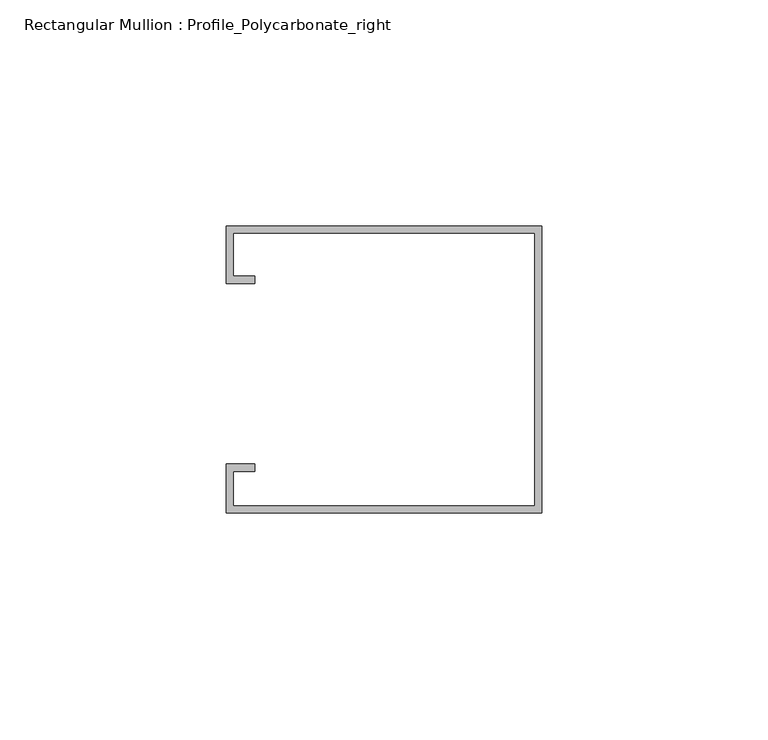
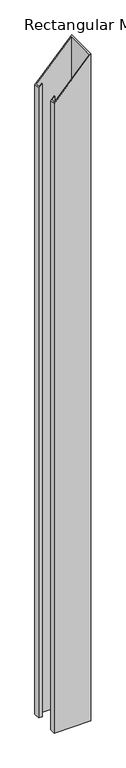
"""IFC4 building model written with IfcOpenShell, lengths in millimetres: member geometry, Rectangular Mullion : Profile_Polycarbonate_right."""

from ifc_helpers import new_model, si_unit, origin, place, context, project, spatial, faceted_brep, source, transform, mapped, element, save


def rectangular_mullion_profile_polycarbonate_right_a4e2f6aa(model_context):
    return source(origin(), model_context, "Body", "Brep", [
        faceted_brep([(0.0, 32.7, -1345.3170334), (0.0, -30.8, -1345.3170334), (-69.85, -30.8, -1345.3170334), (-69.85, -20.0, -1345.3170334), (-63.5, -20.0, -1345.3170334), (-63.5, -21.5875, -1345.3170334), (-68.2625, -21.5875, -1345.3170334), (-68.2625, -29.2125, -1345.3170334), (-1.5875, -29.2125, -1345.3170334), (-1.5875, 31.1125, -1345.3170334), (-68.2625, 31.1125, -1345.3170334), (-68.2625, 21.5875, -1345.3170334), (-63.5, 21.5875, -1345.3170334), (-63.5, 20.0, -1345.3170334), (-69.85, 20.0, -1345.3170334), (-69.85, 32.7, -1345.3170334), (-69.85, 32.7, -75.9129484), (0.0, 32.7, 0.0), (-69.85, 20.0, -75.9129484), (-63.5, 20.0, -69.0117713), (-63.5, 21.5875, -69.0117713), (-68.2625, 21.5875, -74.1876542), (-68.2625, 31.1125, -74.1876542), (-1.5875, 31.1125, -1.7252943), (-1.5875, -29.2125, -1.7252943), (-68.2625, -29.2125, -74.1876542), (-68.2625, -21.5875, -74.1876542), (-63.5, -21.5875, -69.0117713), (-63.5, -20.0, -69.0117713), (-69.85, -20.0, -75.9129484), (-69.85, -30.8, -75.9129484), (0.0, -30.8, 0.0)], [[[0, 1, 2, 3, 4, 5, 6, 7, 8, 9, 10, 11, 12, 13, 14, 15]], [[16, 17, 0, 15]], [[18, 16, 15, 14]], [[19, 18, 14, 13]], [[20, 19, 13, 12]], [[21, 20, 12, 11]], [[22, 21, 11, 10]], [[23, 22, 10, 9]], [[24, 23, 9, 8]], [[25, 24, 8, 7]], [[26, 25, 7, 6]], [[27, 26, 6, 5]], [[28, 27, 5, 4]], [[29, 28, 4, 3]], [[30, 29, 3, 2]], [[31, 30, 2, 1]], [[17, 31, 1, 0]], [[17, 16, 18, 19, 20, 21, 22, 23, 24, 25, 26, 27, 28, 29, 30, 31]]]),
    ])


if __name__ == "__main__":
    model = new_model("IFC4")
    model_context = context("Model", 3, world=origin())
    ifc_project = project(units=[si_unit("LENGTHUNIT", "METRE", prefix="MILLI")], contexts=[model_context])
    site = spatial("IfcSite", under=ifc_project)
    building = spatial("IfcBuilding", under=site)
    placement = place(None, origin())
    rectangular_mullion_profile_polycarbonate_right_shape = rectangular_mullion_profile_polycarbonate_right_a4e2f6aa(model_context)
    element("IfcMember", 1, ObjectType="Rectangular Mullion : Profile_Polycarbonate_right", at=placement, inside=building, context=model_context, shape_type="MappedRepresentation", body=[
        mapped(rectangular_mullion_profile_polycarbonate_right_shape, transform((0.0, 0.0, 0.0), x_axis=(1.0, 0.0, 0.0), y_axis=(0.0, 1.0, 0.0), z_axis=(0.0, 0.0, 1.0))),
    ])
    save(model, "model.ifc")

# Revit data of these elements
# Type "Rectangular Mullion : Profile_Polycarbonate_right"
#   built-in parameter 1007322 = 0.208333 (stored number, unit not read)
#   built-in parameter 1007321 = 0 (stored number, unit not read)
#   built-in parameter 1007320 = 0.00520833 (stored number, unit not read)
# Element 1 (IfcMember, "Rectangular Mullion : Profile_Polycarbonate_right")
#   Materials on its faces: "ALUMINUM PROFILE AT POLYCARBONATE PANEL"
# Materials
#   "ALUMINUM PROFILE AT POLYCARBONATE PANEL": class "Metal", colour RGB 244 244 244, transparency 0, Description = "Aluminum 6061", Cost = 0
